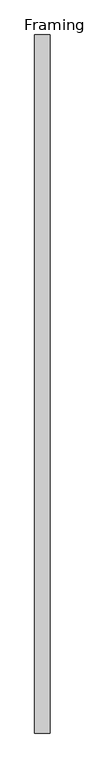
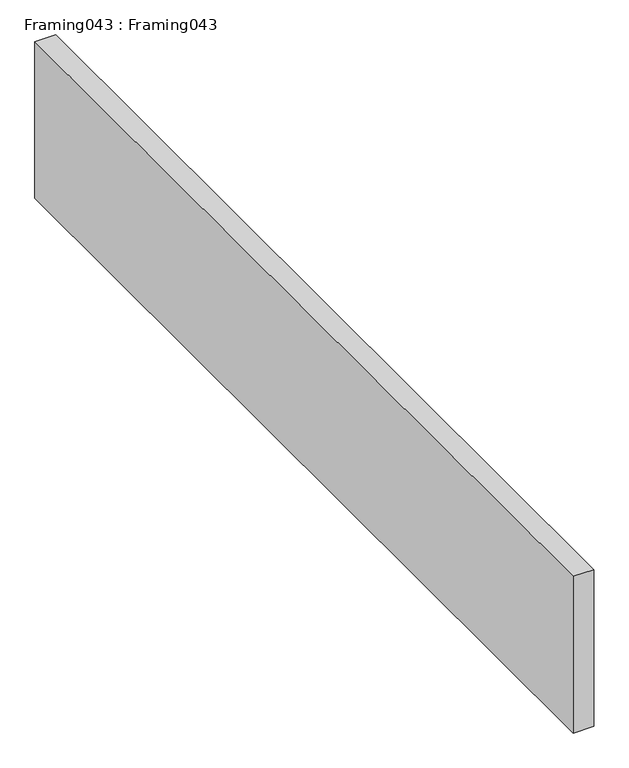
"""IFC4 building model written with IfcOpenShell, lengths in millimetres: proxy geometry, Framing043 : Framing043."""

from ifc_helpers import new_model, si_unit, frame, origin, place, context, project, spatial, polyline, outline, extrude, source, transform, mapped, element, save


def framing043_framing043_95ad604c(model_context):
    return source(origin(), model_context, "Body", "SweptSolid", [
        extrude(outline(polyline([(-5785.399396, 7982.1531721), (-5829.849396, 7982.1531721), (-5829.849396, 9982.1531721), (-5785.399396, 9982.1531721), (-5785.399396, 7982.1531721)])), frame((0.0, 0.0, 43056.1274708), z_axis=(0.0, 0.0, 1.0), x_axis=(1.0, 0.0, 0.0)), (0.0, 0.0, 1.0), 355.2981173),
    ])


if __name__ == "__main__":
    model = new_model("IFC4")
    model_context = context("Model", 3, world=origin())
    ifc_project = project(units=[si_unit("LENGTHUNIT", "METRE", prefix="MILLI")], contexts=[model_context])
    site = spatial("IfcSite", under=ifc_project)
    building = spatial("IfcBuilding", under=site)
    placement = place(None, origin())
    framing043_framing043_shape = framing043_framing043_95ad604c(model_context)
    element("IfcBuildingElementProxy", 1, Name="Framing043 : Framing043", ObjectType="Framing043 : Framing043", at=placement, inside=building, context=model_context, shape_type="MappedRepresentation", body=[
        mapped(framing043_framing043_shape, transform((0.0, 0.0, 0.0), x_axis=(1.0, 0.0, 0.0), y_axis=(0.0, 1.0, 0.0), z_axis=(0.0, 0.0, 1.0))),
    ])
    save(model, "model.ifc")

# Revit data of these elements
# Type "Framing043 : Framing043"
#   NameOverride = "Framing043"
# Element 1 (IfcBuildingElementProxy, "Framing043 : Framing043")
#   Materials on its faces: "WOOD FRAMING (SEE STRUCT DWGS)"
# Materials
#   "WOOD FRAMING (SEE STRUCT DWGS)": class "Unassigned", colour RGB 224 188 168, transparency 0, Cost = 0
